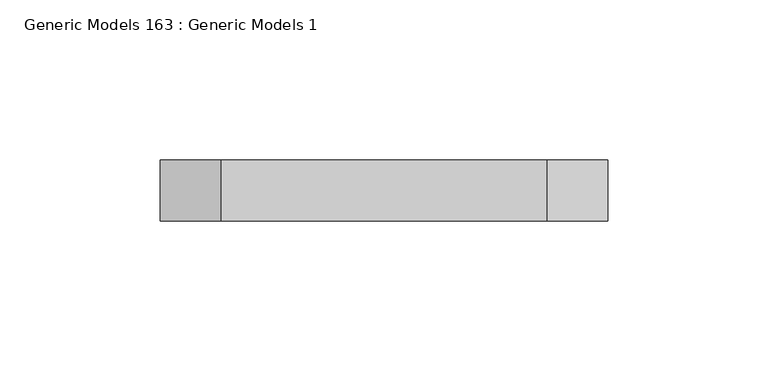
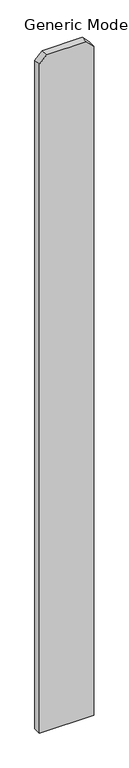
"""IFC4 building model written with IfcOpenShell, lengths in millimetres: proxy geometry, Generic Models 163 : Generic Models 1."""

import ifcopenshell
import ifcopenshell.guid

model = None  # the IFC model being written
_history = None  # IfcOwnerHistory: only IFC2X3 demands one
_inside = {}  # id of a spatial element -> (the spatial element, [elements in it])
_under = {}  # id of a project, library or spatial element -> (it, [spatial elements below it])
_declared = {}  # id of a project -> (the project, [libraries it declares])
_typed = {}  # id of a type object -> (the type object, [elements of that type])
_made_of = {}  # id of a material, layer set ... -> (it, [elements and type objects made of it])


def new_model(schema):
    """Start an empty IFC model of exactly this schema.

    Asked for "IFC4X3", IfcOpenShell would pick the latest addendum, in which some entities
    have other attributes; the version numbers below select the first issue.
    IFC2X3 requires an IfcOwnerHistory on every rooted entity: one is made here for all.
    """
    global model, _history
    if schema == "IFC4X3":
        model = ifcopenshell.file(schema_version=(4, 3, 0, 0))
    else:
        model = ifcopenshell.file(schema=schema)
    _inside.clear()
    _under.clear()
    _declared.clear()
    _typed.clear()
    _made_of.clear()
    _history = None
    if model.schema == "IFC2X3":
        org = make("IfcOrganization", Name="unknown")
        user = make(
            "IfcPersonAndOrganization",
            ThePerson=make("IfcPerson", FamilyName="unknown"),
            TheOrganization=org,
        )
        app = make(
            "IfcApplication",
            ApplicationDeveloper=org,
            Version="unknown",
            ApplicationFullName="unknown",
            ApplicationIdentifier="unknown",
        )
        _history = make(
            "IfcOwnerHistory",
            OwningUser=user,
            OwningApplication=app,
            ChangeAction="ADDED",
            CreationDate=0,
        )
    return model


def make(cls, **values):
    """One entity of the class cls with the attributes given. An attribute that is None is left unset."""
    return model.create_entity(
        cls, **{name: value for name, value in values.items() if value is not None}
    )


def rooted(cls, **values):
    """An entity with a GlobalId (a new one), such as an element, a storey or a relation."""
    return make(cls, GlobalId=ifcopenshell.guid.new(), OwnerHistory=_history, **values)


def si_unit(unit_type, name, prefix=None):
    """IfcSIUnit, for example si_unit("LENGTHUNIT", "METRE", prefix="MILLI")."""
    return make("IfcSIUnit", UnitType=unit_type, Prefix=prefix, Name=name)


def assignment(units):
    """IfcUnitAssignment: the units of a project."""
    return None if units is None else make("IfcUnitAssignment", Units=units)


def point(xyz):
    """IfcCartesianPoint."""
    return None if xyz is None else make("IfcCartesianPoint", Coordinates=xyz)


def direction(xyz):
    """IfcDirection."""
    return None if xyz is None else make("IfcDirection", DirectionRatios=xyz)


def frame(location, z_axis=None, x_axis=None):
    """IfcAxis2Placement3D, a coordinate frame: its origin and axes. An axis left out is left unset."""
    return make(
        "IfcAxis2Placement3D",
        Location=point(location),
        Axis=direction(z_axis),
        RefDirection=direction(x_axis),
    )


def origin():
    """The frame at (0, 0, 0) with its axes left unset."""
    return frame((0.0, 0.0, 0.0))


def place(relative_to, where):
    """IfcLocalPlacement: puts the frame where relative to a parent placement (None: the world)."""
    return make(
        "IfcLocalPlacement", PlacementRelTo=relative_to, RelativePlacement=where
    )


def context(
    kind, dimensions, precision=None, world=None, true_north=None, identifier=None
):
    """IfcGeometricRepresentationContext, for example the 3D "Model" context."""
    return make(
        "IfcGeometricRepresentationContext",
        ContextIdentifier=identifier,
        ContextType=kind,
        CoordinateSpaceDimension=dimensions,
        Precision=precision,
        WorldCoordinateSystem=world,
        TrueNorth=true_north,
    )


def project(units=None, contexts=None):
    """IfcProject with its units and contexts."""
    return rooted(
        "IfcProject",
        Name="project",
        RepresentationContexts=contexts,
        UnitsInContext=assignment(units),
    )


def spatial(cls, under=None, at=None, **own):
    """A site, building, storey or space (cls), placed at a placement, below another one or the project."""
    s = rooted(cls, ObjectPlacement=at, **own)
    if under is not None:
        _under.setdefault(under.id(), (under, []))[1].append(s)
    return s


def polyline(points):
    """IfcPolyline through the points."""
    return make("IfcPolyline", Points=[point(p) for p in points])


def outline(outer, holes=None, kind="AREA"):
    """IfcArbitraryClosedProfileDef: a profile drawn as a closed curve; with holes, ...WithVoids."""
    if holes is None:
        return make("IfcArbitraryClosedProfileDef", ProfileType=kind, OuterCurve=outer)
    return make(
        "IfcArbitraryProfileDefWithVoids",
        ProfileType=kind,
        OuterCurve=outer,
        InnerCurves=holes,
    )


def extrude(swept, where, along, depth):
    """IfcExtrudedAreaSolid: the profile swept, set in the frame where, extruded along a direction by depth."""
    return make(
        "IfcExtrudedAreaSolid",
        SweptArea=swept,
        Position=where,
        ExtrudedDirection=direction(along),
        Depth=depth,
    )


def shape(context_of_items, identifier, shape_type, items):
    """IfcShapeRepresentation: the items that make up one representation, for example the "Body"."""
    return make(
        "IfcShapeRepresentation",
        ContextOfItems=context_of_items,
        RepresentationIdentifier=identifier,
        RepresentationType=shape_type,
        Items=items,
    )


def source(mapping_origin, context_of_items, identifier, shape_type, items):
    """IfcRepresentationMap: a shape defined once, which mapped items show again and again."""
    return make(
        "IfcRepresentationMap",
        MappingOrigin=mapping_origin,
        MappedRepresentation=shape(context_of_items, identifier, shape_type, items),
    )


def transform(
    local_origin,
    x_axis=None,
    y_axis=None,
    z_axis=None,
    scale=None,
    scale2=None,
    scale3=None,
    uniform=True,
):
    """IfcCartesianTransformationOperator3D, or its non-uniform kind. x_axis, y_axis, z_axis: its Axis1, 2, 3."""
    if uniform:
        return make(
            "IfcCartesianTransformationOperator3D",
            Axis1=direction(x_axis),
            Axis2=direction(y_axis),
            LocalOrigin=point(local_origin),
            Scale=scale,
            Axis3=direction(z_axis),
        )
    return make(
        "IfcCartesianTransformationOperator3DnonUniform",
        Axis1=direction(x_axis),
        Axis2=direction(y_axis),
        LocalOrigin=point(local_origin),
        Scale=scale,
        Axis3=direction(z_axis),
        Scale2=scale2,
        Scale3=scale3,
    )


def mapped(mapping_source, mapping_target):
    """IfcMappedItem: shows the shape of a source again, moved by a transform."""
    return make(
        "IfcMappedItem", MappingSource=mapping_source, MappingTarget=mapping_target
    )


def made_of(thing, what):
    """Note that an element or type object is made of a material, layer set ...; save() writes the relation."""
    if what is not None:
        _made_of.setdefault(what.id(), (what, []))[1].append(thing)
    return thing


def element(
    cls,
    number,
    at=None,
    inside=None,
    cuts=None,
    type_object=None,
    material=None,
    context=None,
    identifier="Body",
    shape_type=None,
    held_by="IfcProductDefinitionShape",
    body=None,
    shapes=None,
    **own,
):
    """One element of the class cls, such as IfcWall. Its Tag is "e" and its number.

    at: its placement. inside: the storey or other place that contains it. cuts: it is an
    opening in that element (IfcRelVoidsElement). A single representation is given by context,
    identifier, shape_type and body (its items); several are given by shapes. held_by: the class
    of the entity that holds the representations. save() writes the other relations.
    """
    e = rooted(cls, Tag="e%d" % number, ObjectPlacement=at, **own)
    if body is not None:
        shapes = [shape(context, identifier, shape_type, body)]
    if shapes is not None:
        e.Representation = make(held_by, Representations=shapes)
    if inside is not None:
        _inside.setdefault(inside.id(), (inside, []))[1].append(e)
    if cuts is not None:
        rooted(
            "IfcRelVoidsElement", RelatingBuildingElement=cuts, RelatedOpeningElement=e
        )
    if type_object is not None:
        _typed.setdefault(type_object.id(), (type_object, []))[1].append(e)
    return made_of(e, material)


def aggregate(whole, parts):
    """IfcRelAggregates: a whole, such as a stair, and the parts it consists of."""
    return rooted("IfcRelAggregates", RelatingObject=whole, RelatedObjects=parts)


def save(model, path):
    """Write the relations noted so far, then the file.

    IfcRelAggregates (storeys below a building ...), IfcRelContainedInSpatialStructure (elements
    in a storey), IfcRelDefinesByType, IfcRelAssociatesMaterial and IfcRelDeclares: one each for
    every whole, place, type object, material and project.
    """
    for whole, parts in _under.values():
        aggregate(whole, parts)
    for where, things in _inside.values():
        rooted(
            "IfcRelContainedInSpatialStructure",
            RelatedElements=things,
            RelatingStructure=where,
        )
    for kind, things in _typed.values():
        rooted("IfcRelDefinesByType", RelatedObjects=things, RelatingType=kind)
    for what, things in _made_of.values():
        rooted("IfcRelAssociatesMaterial", RelatedObjects=things, RelatingMaterial=what)
    for by, libraries in _declared.values():
        rooted("IfcRelDeclares", RelatingContext=by, RelatedDefinitions=libraries)
    model.write(path)


def generic_models_163_generic_models_1_4947abff(model_context):
    return source(origin(), model_context, "Body", "SweptSolid", [
        extrude(outline(polyline([(76.2, 54837.0125), (1885.95, 54837.0125), (1905.0, 54817.9625), (1905.0, 54716.3625), (1885.95, 54697.3125), (76.2, 54697.3125), (76.2, 54837.0125)])), frame((0.0, 547.6875, 0.0), z_axis=(0.0, 1.0, 0.0), x_axis=(0.0, 0.0, 1.0)), (0.0, 0.0, 1.0), 19.05),
    ])


if __name__ == "__main__":
    model = new_model("IFC4")
    model_context = context("Model", 3, world=origin())
    ifc_project = project(units=[si_unit("LENGTHUNIT", "METRE", prefix="MILLI")], contexts=[model_context])
    site = spatial("IfcSite", under=ifc_project)
    building = spatial("IfcBuilding", under=site)
    placement = place(None, origin())
    generic_models_163_generic_models_1_shape = generic_models_163_generic_models_1_4947abff(model_context)
    element("IfcBuildingElementProxy", 1, Name="Generic Models 163 : Generic Models 1", ObjectType="Generic Models 163 : Generic Models 1", at=placement, inside=building, context=model_context, shape_type="MappedRepresentation", body=[
        mapped(generic_models_163_generic_models_1_shape, transform((0.0, 0.0, 0.0), x_axis=(1.0, 0.0, 0.0), y_axis=(0.0, 1.0, 0.0), z_axis=(0.0, 0.0, 1.0))),
    ])
    save(model, "model.ifc")

# Revit data of these elements
# Element 1 (IfcBuildingElementProxy, "Generic Models 163 : Generic Models 1")
#   Materials on its faces: "VERTICAL 1X6 CEDAR PLANKS W/ CLEAR WOOD SEALER"
# Materials
#   "VERTICAL 1X6 CEDAR PLANKS W/ CLEAR WOOD SEALER": class "Wood", colour RGB 234 198 147, transparency 0, Description = "Pinus Echinata", Cost = 0
